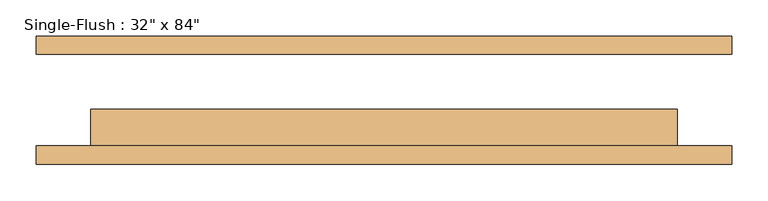
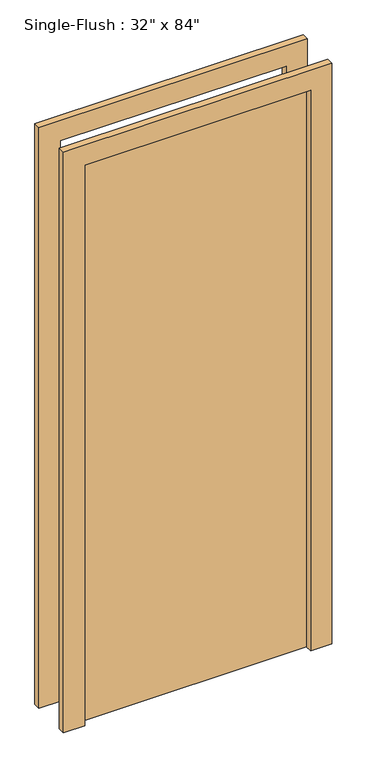
"""IFC4 building model written with IfcOpenShell, lengths in millimetres: door geometry."""

from ifc_helpers import new_model, si_unit, frame, origin, origin_with_axes, place, context, project, spatial, polyline, outline, extrude, source, transform, mapped, element, save


def door_ba4c5d75(model_context):
    return source(origin(), model_context, "Body", "SweptSolid", [
        extrude(outline(polyline([(2209.8, -482.6), (0.0, -482.6), (0.0, -406.4), (2133.6, -406.4), (2133.6, 406.4), (0.0, 406.4), (0.0, 482.6), (2209.8, 482.6), (2209.8, -482.6)])), frame((0.0, -88.9, 0.0), z_axis=(0.0, 1.0, 0.0), x_axis=(0.0, 0.0, 1.0)), (0.0, 0.0, 1.0), 25.4),
        extrude(outline(polyline([(2209.8, 482.6), (2209.8, -482.6), (0.0, -482.6), (0.0, -406.4), (2133.6, -406.4), (2133.6, 406.4), (0.0, 406.4), (0.0, 482.6), (2209.8, 482.6)])), frame((0.0, 63.5, 0.0), z_axis=(0.0, 1.0, 0.0), x_axis=(0.0, 0.0, 1.0)), (0.0, 0.0, 1.0), 25.4),
        extrude(outline(polyline([(406.4, -12.7), (406.4, -63.5), (-406.4, -63.5), (-406.4, -12.7), (406.4, -12.7)])), origin_with_axes(), (0.0, 0.0, 1.0), 2133.6),
    ])


if __name__ == "__main__":
    model = new_model("IFC4")
    model_context = context("Model", 3, world=origin())
    ifc_project = project(units=[si_unit("LENGTHUNIT", "METRE", prefix="MILLI")], contexts=[model_context])
    site = spatial("IfcSite", under=ifc_project)
    building = spatial("IfcBuilding", under=site)
    placement = place(None, origin())
    door_shape = door_ba4c5d75(model_context)
    element("IfcDoor", 1, ObjectType="Single-Flush : 32\" x 84\"", at=placement, inside=building, context=model_context, shape_type="MappedRepresentation", body=[
        mapped(door_shape, transform((0.0, 0.0, 0.0), x_axis=(1.0, 0.0, 0.0), y_axis=(0.0, 1.0, 0.0), z_axis=(0.0, 0.0, 1.0))),
    ])
    save(model, "model.ifc")

# Revit data of these elements
# Type "Single-Flush : 32\" x 84\""
#   Type Mark = "10"
#   Construction Type Id = "MDOOR"
#   Assembly Code = "C1020"
#   Analytic Construction = "Metal"
#   Thickness = 0' - 2"
#   Heat Transfer Coefficient (U) = 3.7021 W/(m²·K)
#   Height = 7' - 0"
#   Trim Projection Ext = 0' - 1"
#   Trim Projection Int = 0' - 1"
#   Trim Width = 0' - 3"
#   Width = 2' - 8"
#   Door Material = Door - Panel
#   Frame Material = Door - Frame
#   Visual Light Transmittance = 0
#   Solar Heat Gain Coefficient = 0
#   Function = (empty or 0)
#   Wall Closure = (empty or 0)
# Element 1 (IfcDoor, "Single-Flush : 32\" x 84\"")
#   Materials on its faces: "Door - Frame", "Door - Panel"
# Materials
#   "Door - Panel": class "Wood", colour RGB 210 159 95, transparency 0
#   "Door - Frame": class "Miscellaneous", colour RGB 118 70 51, transparency 0
